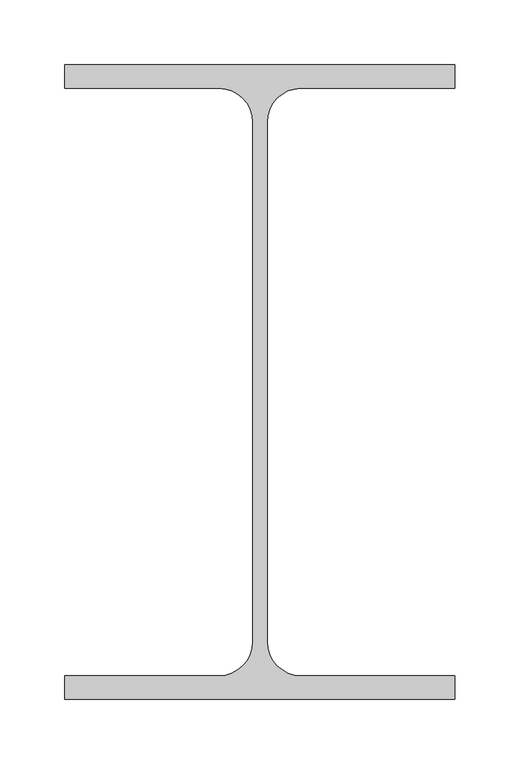
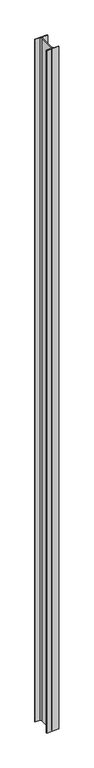
"""IFC4 building model written with IfcOpenShell, lengths in millimetres: column geometry, 0912_Steel Column_H_KSD3502 : H_SC_ASC_H-488x300x11x18."""

from ifc_helpers import new_model, si_unit, point, frame, frame_2d, origin, place, context, project, spatial, polyline, circle_curve, trimmed, segment, composite_curve, outline, extrude, source, transform, mapped, element, save


def column_c3fe6796(model_context):
    return source(origin(), model_context, "Body", "SweptSolid", [
        extrude(outline(composite_curve([segment(polyline([(150.0, 244.0), (150.0, 226.0), (31.5, 226.0)]), True, "CONTINUOUS"), segment(trimmed(circle_curve(frame_2d((31.5, 200.0)), 26.0), [point((31.5, 226.0))], [point((5.5, 200.0))], True, "CARTESIAN"), True, "CONTINUOUS"), segment(polyline([(5.5, 200.0), (5.5, -200.0)]), True, "CONTINUOUS"), segment(trimmed(circle_curve(frame_2d((31.5, -200.0)), 26.0), [point((5.5, -200.0))], [point((31.5, -226.0))], True, "CARTESIAN"), True, "CONTINUOUS"), segment(polyline([(31.5, -226.0), (150.0, -226.0), (150.0, -244.0), (-150.0, -244.0), (-150.0, -226.0), (-31.5, -226.0)]), True, "CONTINUOUS"), segment(trimmed(circle_curve(frame_2d((-31.5, -200.0)), 26.0), [point((-31.5, -226.0))], [point((-5.5, -200.0))], True, "CARTESIAN"), True, "CONTINUOUS"), segment(polyline([(-5.5, -200.0), (-5.5, 200.0)]), True, "CONTINUOUS"), segment(trimmed(circle_curve(frame_2d((-31.5, 200.0)), 26.0), [point((-5.5, 200.0))], [point((-31.5, 226.0))], True, "CARTESIAN"), True, "CONTINUOUS"), segment(polyline([(-31.5, 226.0), (-150.0, 226.0), (-150.0, 244.0), (150.0, 244.0)]), True, "CONTINUOUS")], self_intersect=False)), frame((0.0, 0.0, 685.9720055), z_axis=(0.0, 0.0, 1.0), x_axis=(1.0, 0.0, 0.0)), (0.0, 0.0, 1.0), 17514.0),
    ])


if __name__ == "__main__":
    model = new_model("IFC4")
    model_context = context("Model", 3, world=origin())
    ifc_project = project(units=[si_unit("LENGTHUNIT", "METRE", prefix="MILLI")], contexts=[model_context])
    site = spatial("IfcSite", under=ifc_project)
    building = spatial("IfcBuilding", under=site)
    placement = place(None, origin())
    column_shape = column_c3fe6796(model_context)
    element("IfcColumn", 1, ObjectType="0912_Steel Column_H_KSD3502 : H_SC_ASC_H-488x300x11x18", at=placement, inside=building, context=model_context, shape_type="MappedRepresentation", body=[
        mapped(column_shape, transform((0.0, 0.0, 0.0), x_axis=(1.0, 0.0, 0.0), y_axis=(0.0, 1.0, 0.0), z_axis=(0.0, 0.0, 1.0))),
    ])
    save(model, "model.ifc")

# Revit data of these elements
# Type "0912_Steel Column_H_KSD3502 : H_SC_ASC_H-488x300x11x18"
#   H_WM Code_1 = "S01AA002-00001 | Main Steel Structure Fabrication Work | Shelter/Building | Medium Steel - Standard (90KG/M>Weight≥30KG/M) | Material: (   )"
#   H_WM Code_2 = "S03AA028-00001 | Main Steel Structure Erection Work | Shelter/Building | Medium Steel (90KG/M>Weight≥30KG/M) | Material: (   )"
#   H_WM Code_3 = "S01AA010-00001 | Main Steel Structure Fabrication Work | Shelter/Building | Steel Painting/Coating | for Non-Fireproofed Steel Surface, Surface Preparation, Primer, Second & Final Coat | Material: (   )"
#   H_Q'ty Cal Type Tag = "SC-Q2"
#   Width = 30.0 cm
#   Web Thickness = 1.1 cm
#   Web Fillet = 2.6 cm
#   Warping Constant = 4473230.0 cm⁶
#   Torsional Moment of Inertia = 137.492 cm⁴
#   Section Area = 163.5 cm²
#   Plastic Modulus weak axis = 830.0 cm³
#   Plastic Modulus strong axis = 3230.0 cm³
#   Perimeter = 2.11 m²/m
#   Nominal Weight = 128.00 kgf/m
#   Moment of Inertia weak axis = 8110.00 cm⁴
#   Moment of Inertia strong axis = 71000.00 cm⁴
#   Height = 48.8 cm
#   Flange Thickness = 1.8 cm
#   Elastic Modulus weak axis = 541.0 cm³
#   Elastic Modulus strong axis = 2910.0 cm³
#   Centroid Vertical = 24.4 cm
#   Centroid Horizontal = 15.0 cm
#   Structural Material [instance default] = Steel, 45-345
#   Section Name Key = ""
#   Bolt Spacing = 0
#   Assembly Code = ""
# Element 1 (IfcColumn, "0912_Steel Column_H_KSD3502 : H_SC_ASC_H-488x300x11x18")
#   Structural Material = A03AD029-00005_Anchor Bolt (Installation only)_M24
#   Materials on its faces: "A03AD029-00005_Anchor Bolt (Installation only)_M24"
# Materials
#   "Steel, 45-345": class "Metal", colour RGB 189 187 185, transparency 0, Description = "Steel 345 MPa", Cost = 0
#   "A03AD029-00005_Anchor Bolt (Installation only)_M24": class "Unassigned", colour RGB 84 83 81, transparency 0, Cost = 0
